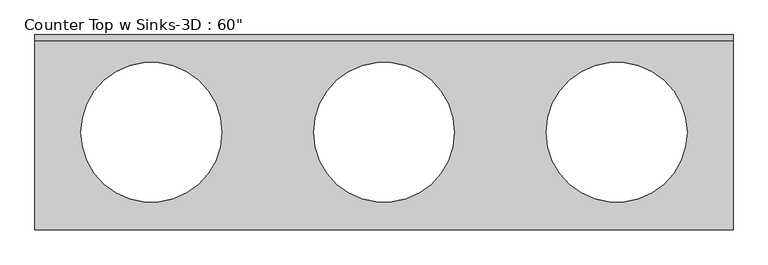
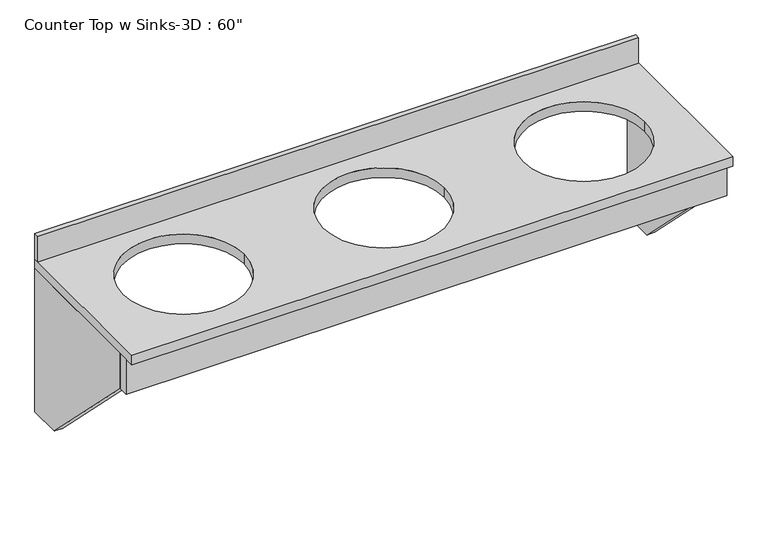
"""IFC4 building model written with IfcOpenShell, lengths in millimetres: furniture geometry."""

import ifcopenshell
import ifcopenshell.guid

model = None  # the IFC model being written
_history = None  # IfcOwnerHistory: only IFC2X3 demands one
_inside = {}  # id of a spatial element -> (the spatial element, [elements in it])
_under = {}  # id of a project, library or spatial element -> (it, [spatial elements below it])
_declared = {}  # id of a project -> (the project, [libraries it declares])
_typed = {}  # id of a type object -> (the type object, [elements of that type])
_made_of = {}  # id of a material, layer set ... -> (it, [elements and type objects made of it])


def new_model(schema):
    """Start an empty IFC model of exactly this schema.

    Asked for "IFC4X3", IfcOpenShell would pick the latest addendum, in which some entities
    have other attributes; the version numbers below select the first issue.
    IFC2X3 requires an IfcOwnerHistory on every rooted entity: one is made here for all.
    """
    global model, _history
    if schema == "IFC4X3":
        model = ifcopenshell.file(schema_version=(4, 3, 0, 0))
    else:
        model = ifcopenshell.file(schema=schema)
    _inside.clear()
    _under.clear()
    _declared.clear()
    _typed.clear()
    _made_of.clear()
    _history = None
    if model.schema == "IFC2X3":
        org = make("IfcOrganization", Name="unknown")
        user = make(
            "IfcPersonAndOrganization",
            ThePerson=make("IfcPerson", FamilyName="unknown"),
            TheOrganization=org,
        )
        app = make(
            "IfcApplication",
            ApplicationDeveloper=org,
            Version="unknown",
            ApplicationFullName="unknown",
            ApplicationIdentifier="unknown",
        )
        _history = make(
            "IfcOwnerHistory",
            OwningUser=user,
            OwningApplication=app,
            ChangeAction="ADDED",
            CreationDate=0,
        )
    return model


def make(cls, **values):
    """One entity of the class cls with the attributes given. An attribute that is None is left unset."""
    return model.create_entity(
        cls, **{name: value for name, value in values.items() if value is not None}
    )


def rooted(cls, **values):
    """An entity with a GlobalId (a new one), such as an element, a storey or a relation."""
    return make(cls, GlobalId=ifcopenshell.guid.new(), OwnerHistory=_history, **values)


def si_unit(unit_type, name, prefix=None):
    """IfcSIUnit, for example si_unit("LENGTHUNIT", "METRE", prefix="MILLI")."""
    return make("IfcSIUnit", UnitType=unit_type, Prefix=prefix, Name=name)


def assignment(units):
    """IfcUnitAssignment: the units of a project."""
    return None if units is None else make("IfcUnitAssignment", Units=units)


def point(xyz):
    """IfcCartesianPoint."""
    return None if xyz is None else make("IfcCartesianPoint", Coordinates=xyz)


def direction(xyz):
    """IfcDirection."""
    return None if xyz is None else make("IfcDirection", DirectionRatios=xyz)


def frame(location, z_axis=None, x_axis=None):
    """IfcAxis2Placement3D, a coordinate frame: its origin and axes. An axis left out is left unset."""
    return make(
        "IfcAxis2Placement3D",
        Location=point(location),
        Axis=direction(z_axis),
        RefDirection=direction(x_axis),
    )


def frame_2d(location, x_axis=None):
    """IfcAxis2Placement2D, a coordinate frame in the plane: its origin and x axis."""
    return make(
        "IfcAxis2Placement2D", Location=point(location), RefDirection=direction(x_axis)
    )


def origin():
    """The frame at (0, 0, 0) with its axes left unset."""
    return frame((0.0, 0.0, 0.0))


def place(relative_to, where):
    """IfcLocalPlacement: puts the frame where relative to a parent placement (None: the world)."""
    return make(
        "IfcLocalPlacement", PlacementRelTo=relative_to, RelativePlacement=where
    )


def context(
    kind, dimensions, precision=None, world=None, true_north=None, identifier=None
):
    """IfcGeometricRepresentationContext, for example the 3D "Model" context."""
    return make(
        "IfcGeometricRepresentationContext",
        ContextIdentifier=identifier,
        ContextType=kind,
        CoordinateSpaceDimension=dimensions,
        Precision=precision,
        WorldCoordinateSystem=world,
        TrueNorth=true_north,
    )


def project(units=None, contexts=None):
    """IfcProject with its units and contexts."""
    return rooted(
        "IfcProject",
        Name="project",
        RepresentationContexts=contexts,
        UnitsInContext=assignment(units),
    )


def spatial(cls, under=None, at=None, **own):
    """A site, building, storey or space (cls), placed at a placement, below another one or the project."""
    s = rooted(cls, ObjectPlacement=at, **own)
    if under is not None:
        _under.setdefault(under.id(), (under, []))[1].append(s)
    return s


def polyline(points):
    """IfcPolyline through the points."""
    return make("IfcPolyline", Points=[point(p) for p in points])


def circle_curve(where, radius):
    """IfcCircle in the frame where."""
    return make("IfcCircle", Position=where, Radius=radius)


def trimmed(basis, trim1, trim2, sense, master):
    """IfcTrimmedCurve: the piece of a basis curve between two trims."""
    return make(
        "IfcTrimmedCurve",
        BasisCurve=basis,
        Trim1=trim1,
        Trim2=trim2,
        SenseAgreement=sense,
        MasterRepresentation=master,
    )


def segment(curve, same_sense, transition):
    """IfcCompositeCurveSegment."""
    return make(
        "IfcCompositeCurveSegment",
        Transition=transition,
        SameSense=same_sense,
        ParentCurve=curve,
    )


def composite_curve(segments, self_intersect=None):
    """IfcCompositeCurve: segments joined end to end."""
    return make("IfcCompositeCurve", Segments=segments, SelfIntersect=self_intersect)


def outline(outer, holes=None, kind="AREA"):
    """IfcArbitraryClosedProfileDef: a profile drawn as a closed curve; with holes, ...WithVoids."""
    if holes is None:
        return make("IfcArbitraryClosedProfileDef", ProfileType=kind, OuterCurve=outer)
    return make(
        "IfcArbitraryProfileDefWithVoids",
        ProfileType=kind,
        OuterCurve=outer,
        InnerCurves=holes,
    )


def extrude(swept, where, along, depth):
    """IfcExtrudedAreaSolid: the profile swept, set in the frame where, extruded along a direction by depth."""
    return make(
        "IfcExtrudedAreaSolid",
        SweptArea=swept,
        Position=where,
        ExtrudedDirection=direction(along),
        Depth=depth,
    )


def shape(context_of_items, identifier, shape_type, items):
    """IfcShapeRepresentation: the items that make up one representation, for example the "Body"."""
    return make(
        "IfcShapeRepresentation",
        ContextOfItems=context_of_items,
        RepresentationIdentifier=identifier,
        RepresentationType=shape_type,
        Items=items,
    )


def source(mapping_origin, context_of_items, identifier, shape_type, items):
    """IfcRepresentationMap: a shape defined once, which mapped items show again and again."""
    return make(
        "IfcRepresentationMap",
        MappingOrigin=mapping_origin,
        MappedRepresentation=shape(context_of_items, identifier, shape_type, items),
    )


def transform(
    local_origin,
    x_axis=None,
    y_axis=None,
    z_axis=None,
    scale=None,
    scale2=None,
    scale3=None,
    uniform=True,
):
    """IfcCartesianTransformationOperator3D, or its non-uniform kind. x_axis, y_axis, z_axis: its Axis1, 2, 3."""
    if uniform:
        return make(
            "IfcCartesianTransformationOperator3D",
            Axis1=direction(x_axis),
            Axis2=direction(y_axis),
            LocalOrigin=point(local_origin),
            Scale=scale,
            Axis3=direction(z_axis),
        )
    return make(
        "IfcCartesianTransformationOperator3DnonUniform",
        Axis1=direction(x_axis),
        Axis2=direction(y_axis),
        LocalOrigin=point(local_origin),
        Scale=scale,
        Axis3=direction(z_axis),
        Scale2=scale2,
        Scale3=scale3,
    )


def mapped(mapping_source, mapping_target):
    """IfcMappedItem: shows the shape of a source again, moved by a transform."""
    return make(
        "IfcMappedItem", MappingSource=mapping_source, MappingTarget=mapping_target
    )


def made_of(thing, what):
    """Note that an element or type object is made of a material, layer set ...; save() writes the relation."""
    if what is not None:
        _made_of.setdefault(what.id(), (what, []))[1].append(thing)
    return thing


def element(
    cls,
    number,
    at=None,
    inside=None,
    cuts=None,
    type_object=None,
    material=None,
    context=None,
    identifier="Body",
    shape_type=None,
    held_by="IfcProductDefinitionShape",
    body=None,
    shapes=None,
    **own,
):
    """One element of the class cls, such as IfcWall. Its Tag is "e" and its number.

    at: its placement. inside: the storey or other place that contains it. cuts: it is an
    opening in that element (IfcRelVoidsElement). A single representation is given by context,
    identifier, shape_type and body (its items); several are given by shapes. held_by: the class
    of the entity that holds the representations. save() writes the other relations.
    """
    e = rooted(cls, Tag="e%d" % number, ObjectPlacement=at, **own)
    if body is not None:
        shapes = [shape(context, identifier, shape_type, body)]
    if shapes is not None:
        e.Representation = make(held_by, Representations=shapes)
    if inside is not None:
        _inside.setdefault(inside.id(), (inside, []))[1].append(e)
    if cuts is not None:
        rooted(
            "IfcRelVoidsElement", RelatingBuildingElement=cuts, RelatedOpeningElement=e
        )
    if type_object is not None:
        _typed.setdefault(type_object.id(), (type_object, []))[1].append(e)
    return made_of(e, material)


def aggregate(whole, parts):
    """IfcRelAggregates: a whole, such as a stair, and the parts it consists of."""
    return rooted("IfcRelAggregates", RelatingObject=whole, RelatedObjects=parts)


def save(model, path):
    """Write the relations noted so far, then the file.

    IfcRelAggregates (storeys below a building ...), IfcRelContainedInSpatialStructure (elements
    in a storey), IfcRelDefinesByType, IfcRelAssociatesMaterial and IfcRelDeclares: one each for
    every whole, place, type object, material and project.
    """
    for whole, parts in _under.values():
        aggregate(whole, parts)
    for where, things in _inside.values():
        rooted(
            "IfcRelContainedInSpatialStructure",
            RelatedElements=things,
            RelatingStructure=where,
        )
    for kind, things in _typed.values():
        rooted("IfcRelDefinesByType", RelatedObjects=things, RelatingType=kind)
    for what, things in _made_of.values():
        rooted("IfcRelAssociatesMaterial", RelatedObjects=things, RelatingMaterial=what)
    for by, libraries in _declared.values():
        rooted("IfcRelDeclares", RelatingContext=by, RelatedDefinitions=libraries)
    model.write(path)


def furniture_ec8beb64(model_context):
    return source(origin(), model_context, "Body", "SweptSolid", [
        extrude(outline(polyline([(-198.4375, 825.5), (-198.4375, 254.0), (-325.4375, 254.0), (-757.2375, 685.8), (-757.2375, 825.5), (-198.4375, 825.5)])), frame((-1116.1103038, 0.0, 0.0), z_axis=(1.0, 0.0, 0.0), x_axis=(0.0, 1.0, 0.0)), (0.0, 0.0, 1.0), 31.75),
        extrude(outline(polyline([(-198.4375, 825.5), (-198.4375, 254.0), (-325.4375, 254.0), (-757.2375, 685.8), (-757.2375, 825.5), (-198.4375, 825.5)])), frame((1122.2646962, 0.0, 0.0), z_axis=(1.0, 0.0, 0.0), x_axis=(0.0, 1.0, 0.0)), (0.0, 0.0, 1.0), 31.75),
        extrude(outline(polyline([(-1116.1103038, -757.2375), (1154.0146962, -757.2375), (1154.0146962, -795.3375), (-1116.1103038, -795.3375), (-1116.1103038, -757.2375)])), frame((0.0, 0.0, 685.8), z_axis=(0.0, 0.0, 1.0), x_axis=(1.0, 0.0, 0.0)), (0.0, 0.0, 1.0), 139.7),
        extrude(outline(polyline([(1154.0146962, -198.4375), (1154.0146962, -217.4875), (-1116.1103038, -217.4875), (-1116.1103038, -198.4375), (1154.0146962, -198.4375)])), frame((0.0, 0.0, 863.6), z_axis=(0.0, 0.0, 1.0), x_axis=(1.0, 0.0, 0.0)), (0.0, 0.0, 1.0), 101.6),
        extrude(outline(polyline([(1154.0146962, -198.4375), (1154.0146962, -833.4375), (-1116.1103038, -833.4375), (-1116.1103038, -198.4375), (1154.0146962, -198.4375)]), holes=[composite_curve([segment(trimmed(circle_curve(frame_2d((-737.7561371, -515.9375)), 228.6), [point((-966.3561371, -515.9375))], [point((-509.1561371, -515.9375))], True, "CARTESIAN"), True, "CONTINUOUS"), segment(trimmed(circle_curve(frame_2d((-737.7561371, -515.9375)), 228.6), [point((-509.1561371, -515.9375))], [point((-966.3561371, -515.9375))], True, "CARTESIAN"), True, "CONTINUOUS")], self_intersect=False), composite_curve([segment(trimmed(circle_curve(frame_2d((775.6605295, -515.9375)), 228.6), [point((547.0605295, -515.9375))], [point((1004.2605295, -515.9375))], True, "CARTESIAN"), True, "CONTINUOUS"), segment(trimmed(circle_curve(frame_2d((775.6605295, -515.9375)), 228.6), [point((1004.2605295, -515.9375))], [point((547.0605295, -515.9375))], True, "CARTESIAN"), True, "CONTINUOUS")], self_intersect=False), composite_curve([segment(trimmed(circle_curve(frame_2d((18.9521962, -515.9375)), 228.6), [point((-209.6478038, -515.9375))], [point((247.5521962, -515.9375))], True, "CARTESIAN"), True, "CONTINUOUS"), segment(trimmed(circle_curve(frame_2d((18.9521962, -515.9375)), 228.6), [point((247.5521962, -515.9375))], [point((-209.6478038, -515.9375))], True, "CARTESIAN"), True, "CONTINUOUS")], self_intersect=False)]), frame((0.0, 0.0, 825.5), z_axis=(0.0, 0.0, 1.0), x_axis=(1.0, 0.0, 0.0)), (0.0, 0.0, 1.0), 38.1),
    ])


if __name__ == "__main__":
    model = new_model("IFC4")
    model_context = context("Model", 3, world=origin())
    ifc_project = project(units=[si_unit("LENGTHUNIT", "METRE", prefix="MILLI")], contexts=[model_context])
    site = spatial("IfcSite", under=ifc_project)
    building = spatial("IfcBuilding", under=site)
    placement = place(None, origin())
    furniture_shape = furniture_ec8beb64(model_context)
    element("IfcFurniture", 1, ObjectType="Counter Top w Sinks-3D : 60\"", at=placement, inside=building, context=model_context, shape_type="MappedRepresentation", body=[
        mapped(furniture_shape, transform((0.0, 0.0, 0.0), x_axis=(1.0, 0.0, 0.0), y_axis=(0.0, 1.0, 0.0), z_axis=(0.0, 0.0, 1.0))),
    ])
    save(model, "model.ifc")

# Revit data of these elements
# Type "Counter Top w Sinks-3D : 60\""
#   Assembly Code = "C1030400"
#   Height = 2' - 10"
#   Distance To Sink Center [instance default] = 1' - 3"
#   Clear Space = 2' - 3"
#   Counter Thickness = 0' - 1 1/2"
#   Depth = 2' - 1"
#   Length [instance default] = 5' - 0"
#   Number Of Sinks [instance default] = 2
#   Counter Top Material = Counter Top
#   Base Material = Laminate
#   Default Elevation = 0
# Element 1 (IfcFurniture, "Counter Top w Sinks-3D : 60\"")
#   Distance To Sink Center = 1' - 2.89583"
#   Length = 7' - 5 3/8"
#   Number Of Sinks = 3
#   Materials on its faces: "Counter Top", "Laminate"
# Materials
#   "Counter Top": class "Unassigned", colour RGB 247 247 239, transparency 0
#   "Laminate": class "Unassigned", colour RGB 247 235 201, transparency 0
